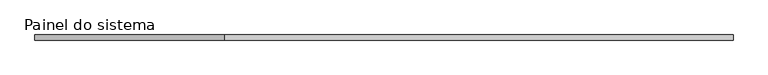
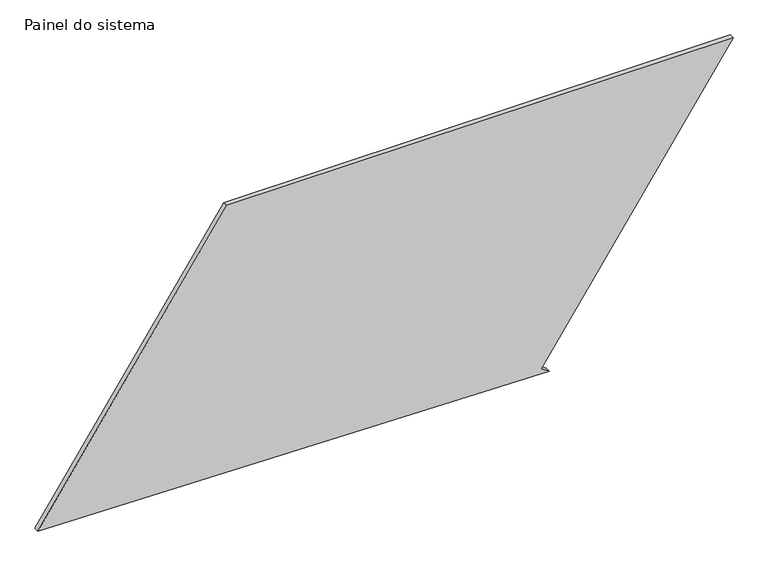
"""IFC4 building model written with IfcOpenShell, lengths in millimetres: plate geometry, Painel do sistema : Envidraçado."""

from ifc_helpers import new_model, si_unit, frame, origin, place, context, project, spatial, polyline, outline, extrude, source, transform, mapped, element, save


def painel_do_sistema_f7516a75(model_context):
    return source(origin(), model_context, "Body", "SweptSolid", [
        extrude(outline(polyline([(0.0, 807.304601), (28.104906, 765.9510732), (1419.8423689, 1711.8111385), (1419.8423689, -781.1506524), (50.46955, -1711.8111385), (0.0, 807.304601)])), frame((0.0, 24.5, 0.0), z_axis=(0.0, 1.0, 0.0), x_axis=(0.0, 0.0, 1.0)), (0.0, 0.0, 1.0), 25.0),
    ])


if __name__ == "__main__":
    model = new_model("IFC4")
    model_context = context("Model", 3, world=origin())
    ifc_project = project(units=[si_unit("LENGTHUNIT", "METRE", prefix="MILLI")], contexts=[model_context])
    site = spatial("IfcSite", under=ifc_project)
    building = spatial("IfcBuilding", under=site)
    placement = place(None, origin())
    painel_do_sistema_shape = painel_do_sistema_f7516a75(model_context)
    element("IfcPlate", 1, ObjectType="Painel do sistema : Envidraçado", at=placement, inside=building, context=model_context, shape_type="MappedRepresentation", body=[
        mapped(painel_do_sistema_shape, transform((0.0, 0.0, 0.0), x_axis=(1.0, 0.0, 0.0), y_axis=(0.0, 1.0, 0.0), z_axis=(0.0, 0.0, 1.0))),
    ])
    save(model, "model.ifc")

# Revit data of these elements
# Type "Painel do sistema : Envidraçado"
#   Construction Type Id = "GSP4R"
#   Analytic Construction = "Vidraça única Pilkington 1/8 pol"
#   Visual Light Transmittance = 0.9
#   Solar Heat Gain Coefficient = 0.86
#   Heat Transfer Coefficient (U) = 6.7069 W/(m²·K)
# Element 1 (IfcPlate, "Painel do sistema : Envidraçado")
#   Materials on its faces: "Vidro"
# Materials
#   "Vidro": class "Vidro", colour RGB 0 128 192, transparency 0.9, Description = "Vidro de sílica", Cost = 0
